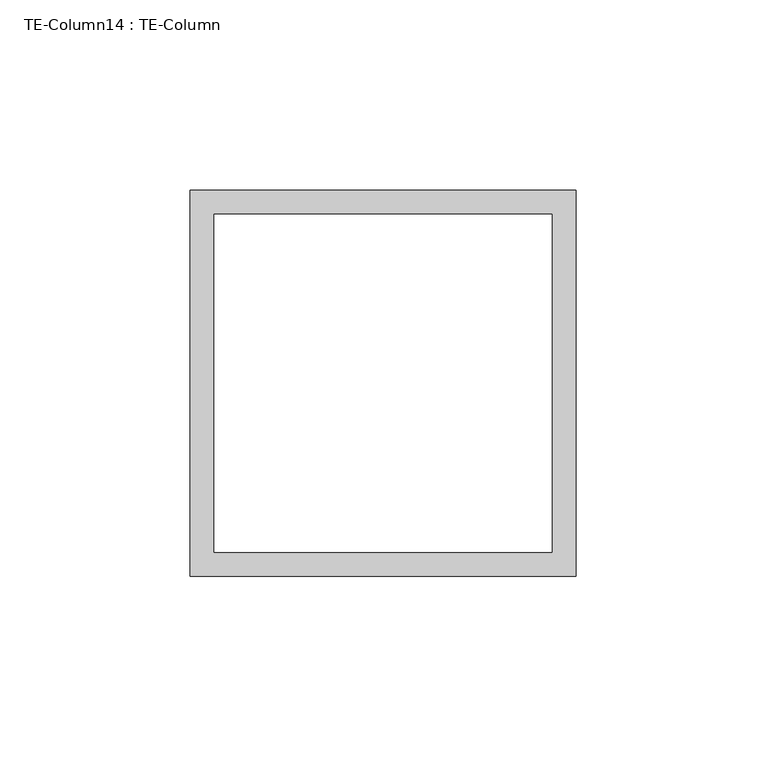
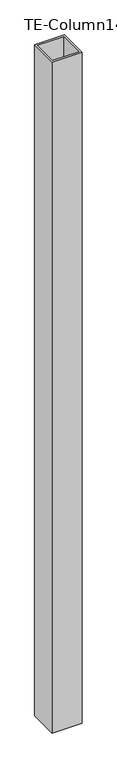
"""IFC4 building model written with IfcOpenShell, lengths in millimetres: proxy geometry, TE-Column14 : TE-Column."""

from ifc_helpers import new_model, si_unit, frame, origin, place, context, project, spatial, polyline, outline, extrude, source, transform, mapped, element, save


def te_column14_te_column_f065ebbf(model_context):
    return source(origin(), model_context, "Body", "SweptSolid", [
        extrude(outline(polyline([(590318.6434739, -532931.4413841), (590217.0434739, -532931.4413841), (590217.0434739, -532829.8413841), (590318.6434739, -532829.8413841), (590318.6434739, -532931.4413841)]), holes=[polyline([(590312.2934739, -532836.1913841), (590223.3934739, -532836.1913841), (590223.3934739, -532925.0913841), (590312.2934739, -532925.0913841), (590312.2934739, -532836.1913841)])]), frame((0.0, 0.0, 28.575), z_axis=(0.0, 0.0, 1.0), x_axis=(1.0, 0.0, 0.0)), (0.0, 0.0, 1.0), 2406.65),
    ])


if __name__ == "__main__":
    model = new_model("IFC4")
    model_context = context("Model", 3, world=origin())
    ifc_project = project(units=[si_unit("LENGTHUNIT", "METRE", prefix="MILLI")], contexts=[model_context])
    site = spatial("IfcSite", under=ifc_project)
    building = spatial("IfcBuilding", under=site)
    placement = place(None, origin())
    te_column14_te_column_shape = te_column14_te_column_f065ebbf(model_context)
    element("IfcBuildingElementProxy", 1, Name="TE-Column14 : TE-Column", ObjectType="TE-Column14 : TE-Column", at=placement, inside=building, context=model_context, shape_type="MappedRepresentation", body=[
        mapped(te_column14_te_column_shape, transform((0.0, 0.0, 0.0), x_axis=(1.0, 0.0, 0.0), y_axis=(0.0, 1.0, 0.0), z_axis=(0.0, 0.0, 1.0))),
    ])
    save(model, "model.ifc")

# Revit data of these elements
# Element 1 (IfcBuildingElementProxy, "TE-Column14 : TE-Column")
#   Materials on its faces: "4\"X4\" GALV. HSS TUBING"
# Materials
#   "4\"X4\" GALV. HSS TUBING": class "Generic", colour RGB 211 211 207, transparency 0, Cost = 0
